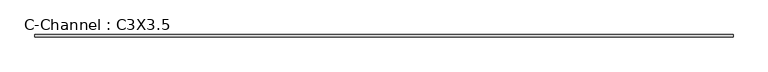
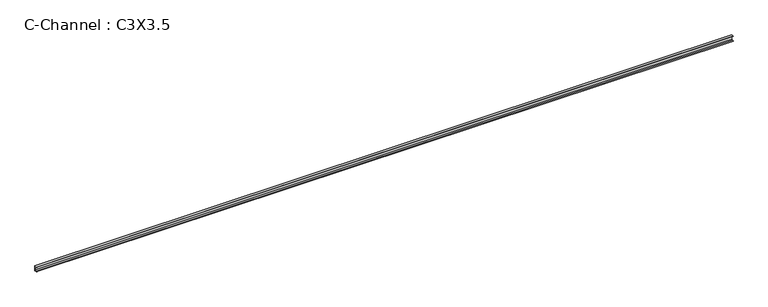
"""IFC4 building model written with IfcOpenShell, lengths in millimetres: beam geometry, C-Channel : C3X3.5."""

from ifc_helpers import new_model, si_unit, point, frame, frame_2d, origin, place, context, project, spatial, polyline, circle_curve, trimmed, segment, composite_curve, outline, extrude, source, transform, mapped, element, save


def c_channel_c3x3_5_2f9156fb(model_context):
    return source(origin(), model_context, "Body", "SweptSolid", [
        extrude(outline(composite_curve([segment(polyline([(11.2522, 38.1), (11.2522, -38.1), (-23.5458, -38.1)]), True, "CONTINUOUS"), segment(trimmed(circle_curve(frame_2d((-16.6116, -38.1)), 6.9342), [point((-23.5458, -38.1))], [point((-16.6116, -31.1658))], False, "CARTESIAN"), True, "CONTINUOUS"), segment(polyline([(-16.6116, -31.1658), (7.8994, -27.283639), (7.8994, 27.283639), (-16.6116, 31.1658)]), True, "CONTINUOUS"), segment(trimmed(circle_curve(frame_2d((-16.6116, 38.1)), 6.9342), [point((-16.6116, 31.1658))], [point((-23.5458, 38.1))], False, "CARTESIAN"), True, "CONTINUOUS"), segment(polyline([(-23.5458, 38.1), (11.2522, 38.1)]), True, "CONTINUOUS")], self_intersect=False)), frame((-5183.4605132, 0.0, 0.0), z_axis=(1.0, 0.0, 0.0), x_axis=(0.0, 1.0, 0.0)), (0.0, 0.0, 1.0), 10366.9210264),
    ])


if __name__ == "__main__":
    model = new_model("IFC4")
    model_context = context("Model", 3, world=origin())
    ifc_project = project(units=[si_unit("LENGTHUNIT", "METRE", prefix="MILLI")], contexts=[model_context])
    site = spatial("IfcSite", under=ifc_project)
    building = spatial("IfcBuilding", under=site)
    placement = place(None, origin())
    c_channel_c3x3_5_shape = c_channel_c3x3_5_2f9156fb(model_context)
    element("IfcBeam", 1, ObjectType="C-Channel : C3X3.5", at=placement, inside=building, context=model_context, shape_type="MappedRepresentation", body=[
        mapped(c_channel_c3x3_5_shape, transform((0.0, 0.0, 0.0), x_axis=(1.0, 0.0, 0.0), y_axis=(0.0, 1.0, 0.0), z_axis=(0.0, 0.0, 1.0))),
    ])
    save(model, "model.ifc")

# Revit data of these elements
# Type "C-Channel : C3X3.5"
#   Assembly Code = "B10"
#   W = 3.5
#   Length [instance default] = 5' - 0"
#   bf = 0' - 1.37"
#   d = 0' - 3"
#   tf = 0' - 0.273"
#   tw = 0' - 0.132"
#   x = 0' - 0.443"
#   A = 0.00756944 SF
#   Structural Material [instance default] = Steel ASTM A36
# Element 1 (IfcBeam, "C-Channel : C3X3.5")
#   Materials on its faces: "Steel ASTM A36"
# Materials
#   "Steel ASTM A36": class "Metal", colour RGB 199 199 199, transparency 0, Description = "Structural steel, ASTM A36 Grade B, mill finish", Cost = 0
